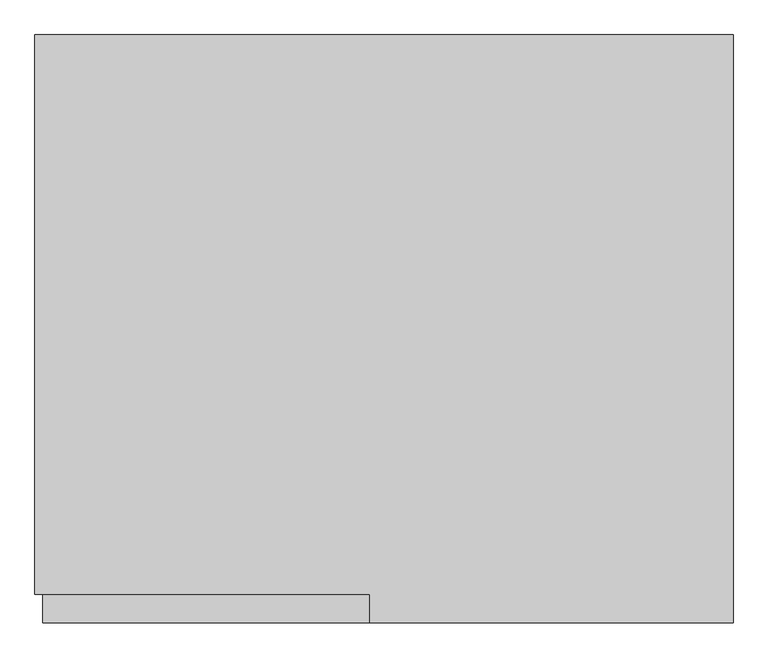
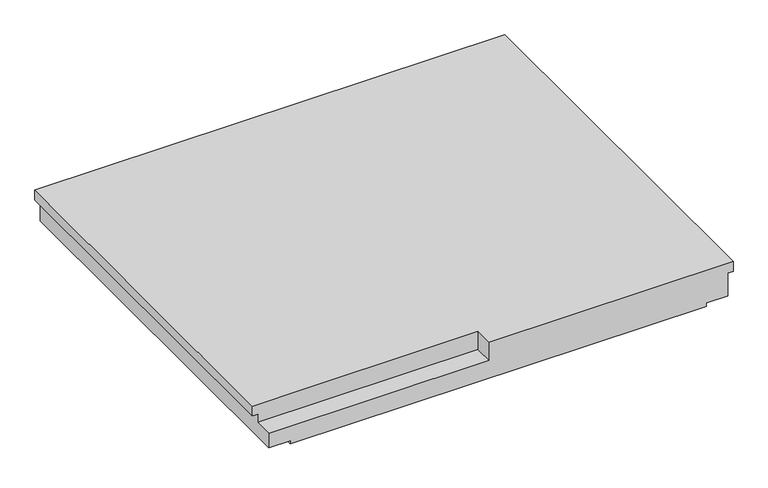
"""IFC4 building model written with IfcOpenShell, lengths in millimetres: stair geometry, NLRS_24_GM_UN_rechthoekig bordes prefab zonder oplegnok-AV_gen_rsf : prefab bordes_gen__2300x2730."""

from ifc_helpers import new_model, si_unit, origin, place, context, project, spatial, faceted_brep, source, transform, mapped, element, save


def stair_f79be4d1(model_context):
    return source(origin(), model_context, "Body", "Brep", [
        faceted_brep([(1365.0, -2300.0, 0.0), (1365.0, -2300.0, -60.0), (1365.0, 0.0, -60.0), (1365.0, 0.0, 0.0), (-55.0, -2300.0, 0.0), (-55.0, -2190.0, 0.0), (-55.0, -2190.0, -110.0), (-55.0, -2300.0, -110.0), (-1365.0, 0.0, 0.0), (-1365.0, 0.0, -60.0), (-1365.0, -2190.0, -60.0), (-1365.0, -2190.0, 0.0), (-1335.0, -2300.0, -110.0), (-1335.0, -2300.0, -200.0), (-1210.0, -2300.0, -200.0), (-1210.0, -2300.0, -220.0), (1210.0, -2300.0, -220.0), (1210.0, -2300.0, -200.0), (1335.0, -2300.0, -200.0), (1335.0, -2300.0, -60.0), (-1335.0, -2190.0, -110.0), (-1335.0, -2190.0, -60.0), (1335.0, 0.0, -60.0), (1335.0, 0.0, -200.0), (1210.0, 0.0, -200.0), (1210.0, 0.0, -220.0), (-1210.0, 0.0, -220.0), (-1210.0, 0.0, -200.0), (-1335.0, 0.0, -200.0), (-1335.0, 0.0, -60.0)], [[[0, 1, 2, 3]], [[4, 5, 6, 7]], [[8, 9, 10, 11]], [[12, 13, 14, 15, 16, 17, 18, 19, 1, 0, 4, 7]], [[7, 6, 20, 12]], [[11, 10, 21, 20, 6, 5]], [[11, 5, 4, 0, 3, 8]], [[8, 3, 2, 22, 23, 24, 25, 26, 27, 28, 29, 9]], [[26, 25, 16, 15]], [[21, 10, 9, 29]], [[13, 12, 20, 21, 29, 28]], [[28, 27, 14, 13]], [[27, 26, 15, 14]], [[22, 2, 1, 19]], [[19, 18, 23, 22]], [[18, 17, 24, 23]], [[17, 16, 25, 24]]]),
    ])


if __name__ == "__main__":
    model = new_model("IFC4")
    model_context = context("Model", 3, world=origin())
    ifc_project = project(units=[si_unit("LENGTHUNIT", "METRE", prefix="MILLI")], contexts=[model_context])
    site = spatial("IfcSite", under=ifc_project)
    building = spatial("IfcBuilding", under=site)
    placement = place(None, origin())
    stair_shape = stair_f79be4d1(model_context)
    element("IfcStair", 1, ObjectType="NLRS_24_GM_UN_rechthoekig bordes prefab zonder oplegnok-AV_gen_rsf : prefab bordes_gen__2300x2730", at=placement, inside=building, context=model_context, shape_type="MappedRepresentation", body=[
        mapped(stair_shape, transform((0.0, 0.0, 0.0), x_axis=(1.0, 0.0, 0.0), y_axis=(0.0, 1.0, 0.0), z_axis=(0.0, 0.0, 1.0))),
    ])
    save(model, "model.ifc")

# Revit data of these elements
# Type "NLRS_24_GM_UN_rechthoekig bordes prefab zonder oplegnok-AV_gen_rsf : prefab bordes_gen__2300x2730"
#   IfcExportAs = "IfcStair"
#   Type Comments = " "
#   Model = " "
#   Manufacturer = " "
#   Description = "rechthoekig bordes prefab\r\n1930x4395"
#   Assembly Code = "24.15"
#   Width = 2730 mm
#   Thickness = 220 mm
#   Perimeter = 10060 mm
#   NLRS_C_lengte_02 = 1310 mm
#   NLRS_C_lengte_01 = 1310 mm
#   NLRS_C_hoogte_02 = 110 mm
#   NLRS_C_hoogte_01 = 110 mm
#   NLRS_C_diepte_04 = 2300 mm
#   NLRS_C_diepte_03 = 2300 mm
#   NLRS_C_diepte_02 = 110 mm
#   NLRS_C_diepte_01 = 110 mm
#   Length = 2300 mm
#   Default Elevation = 1219.2 mm
#   Area = 6.279 m²
#   NLRS_C_materiaal = NLRS_f2_beton prefab_gen_rsf
#   Keynote = ""
# Element 1 (IfcStair, "NLRS_24_GM_UN_rechthoekig bordes prefab zonder oplegnok-AV_gen_rsf : prefab bordes_gen__2300x2730")
#   Materials on its faces: "NLRS_f2_beton prefab_gen_rsf"
# Materials
#   "NLRS_f2_beton prefab_gen_rsf": class "F - Niet gebakken kunststeen", colour RGB 129 133 118, transparency 0, Keynote = "f2", Manufacturer = "Revit Standards Foundation", URL = "www.revitstandards.org", Description = "beton prefab", Cost = 0
